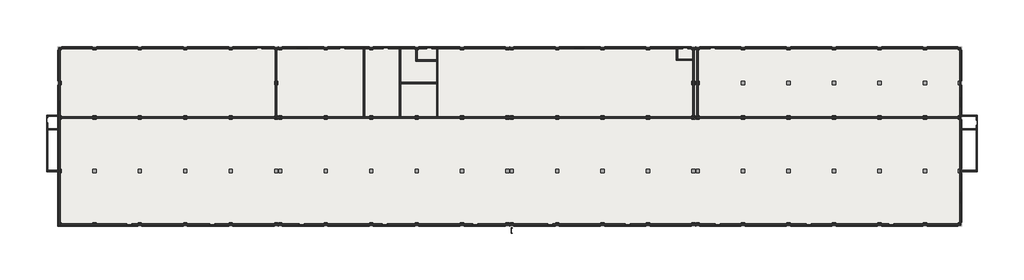
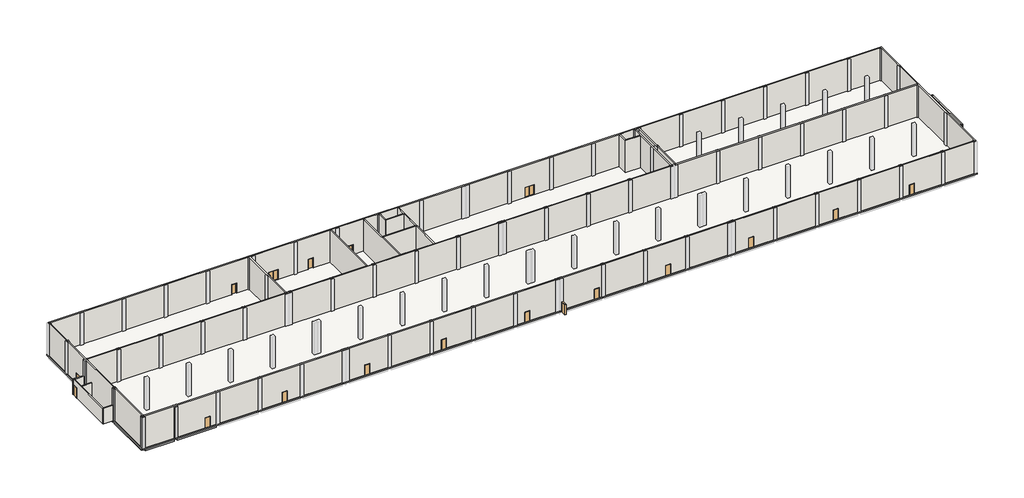
# One storey, part 1 of 4: 27 walls, 24 doors, 4 beams, 4 columns, 1 slab.
"""IFC4 building model written with IfcOpenShell, lengths in millimetres."""

import ifcopenshell
import ifcopenshell.guid

model = None  # the IFC model being written
_history = None  # IfcOwnerHistory: only IFC2X3 demands one
_inside = {}  # id of a spatial element -> (the spatial element, [elements in it])
_under = {}  # id of a project, library or spatial element -> (it, [spatial elements below it])
_declared = {}  # id of a project -> (the project, [libraries it declares])
_typed = {}  # id of a type object -> (the type object, [elements of that type])
_made_of = {}  # id of a material, layer set ... -> (it, [elements and type objects made of it])


def new_model(schema):
    """Start an empty IFC model of exactly this schema.

    Asked for "IFC4X3", IfcOpenShell would pick the latest addendum, in which some entities
    have other attributes; the version numbers below select the first issue.
    IFC2X3 requires an IfcOwnerHistory on every rooted entity: one is made here for all.
    """
    global model, _history
    if schema == "IFC4X3":
        model = ifcopenshell.file(schema_version=(4, 3, 0, 0))
    else:
        model = ifcopenshell.file(schema=schema)
    _inside.clear()
    _under.clear()
    _declared.clear()
    _typed.clear()
    _made_of.clear()
    _history = None
    if model.schema == "IFC2X3":
        org = make("IfcOrganization", Name="unknown")
        user = make(
            "IfcPersonAndOrganization",
            ThePerson=make("IfcPerson", FamilyName="unknown"),
            TheOrganization=org,
        )
        app = make(
            "IfcApplication",
            ApplicationDeveloper=org,
            Version="unknown",
            ApplicationFullName="unknown",
            ApplicationIdentifier="unknown",
        )
        _history = make(
            "IfcOwnerHistory",
            OwningUser=user,
            OwningApplication=app,
            ChangeAction="ADDED",
            CreationDate=0,
        )
    return model


def make(cls, **values):
    """One entity of the class cls with the attributes given. An attribute that is None is left unset."""
    return model.create_entity(
        cls, **{name: value for name, value in values.items() if value is not None}
    )


def rooted(cls, **values):
    """An entity with a GlobalId (a new one), such as an element, a storey or a relation."""
    return make(cls, GlobalId=ifcopenshell.guid.new(), OwnerHistory=_history, **values)


def si_unit(unit_type, name, prefix=None):
    """IfcSIUnit, for example si_unit("LENGTHUNIT", "METRE", prefix="MILLI")."""
    return make("IfcSIUnit", UnitType=unit_type, Prefix=prefix, Name=name)


def assignment(units):
    """IfcUnitAssignment: the units of a project."""
    return None if units is None else make("IfcUnitAssignment", Units=units)


def point(xyz):
    """IfcCartesianPoint."""
    return None if xyz is None else make("IfcCartesianPoint", Coordinates=xyz)


def direction(xyz):
    """IfcDirection."""
    return None if xyz is None else make("IfcDirection", DirectionRatios=xyz)


def frame(location, z_axis=None, x_axis=None):
    """IfcAxis2Placement3D, a coordinate frame: its origin and axes. An axis left out is left unset."""
    return make(
        "IfcAxis2Placement3D",
        Location=point(location),
        Axis=direction(z_axis),
        RefDirection=direction(x_axis),
    )


def origin():
    """The frame at (0, 0, 0) with its axes left unset."""
    return frame((0.0, 0.0, 0.0))


def origin_with_axes():
    """The frame at (0, 0, 0) with the z axis (0, 0, 1) and the x axis (1, 0, 0) written out."""
    return frame((0.0, 0.0, 0.0), z_axis=(0.0, 0.0, 1.0), x_axis=(1.0, 0.0, 0.0))


def place(relative_to, where):
    """IfcLocalPlacement: puts the frame where relative to a parent placement (None: the world)."""
    return make(
        "IfcLocalPlacement", PlacementRelTo=relative_to, RelativePlacement=where
    )


def context(
    kind, dimensions, precision=None, world=None, true_north=None, identifier=None
):
    """IfcGeometricRepresentationContext, for example the 3D "Model" context."""
    return make(
        "IfcGeometricRepresentationContext",
        ContextIdentifier=identifier,
        ContextType=kind,
        CoordinateSpaceDimension=dimensions,
        Precision=precision,
        WorldCoordinateSystem=world,
        TrueNorth=true_north,
    )


def project(units=None, contexts=None):
    """IfcProject with its units and contexts."""
    return rooted(
        "IfcProject",
        Name="project",
        RepresentationContexts=contexts,
        UnitsInContext=assignment(units),
    )


def spatial(cls, under=None, at=None, **own):
    """A site, building, storey or space (cls), placed at a placement, below another one or the project."""
    s = rooted(cls, ObjectPlacement=at, **own)
    if under is not None:
        _under.setdefault(under.id(), (under, []))[1].append(s)
    return s


def polyline(points):
    """IfcPolyline through the points."""
    return make("IfcPolyline", Points=[point(p) for p in points])


def outline(outer, holes=None, kind="AREA"):
    """IfcArbitraryClosedProfileDef: a profile drawn as a closed curve; with holes, ...WithVoids."""
    if holes is None:
        return make("IfcArbitraryClosedProfileDef", ProfileType=kind, OuterCurve=outer)
    return make(
        "IfcArbitraryProfileDefWithVoids",
        ProfileType=kind,
        OuterCurve=outer,
        InnerCurves=holes,
    )


def extrude(swept, where, along, depth):
    """IfcExtrudedAreaSolid: the profile swept, set in the frame where, extruded along a direction by depth."""
    return make(
        "IfcExtrudedAreaSolid",
        SweptArea=swept,
        Position=where,
        ExtrudedDirection=direction(along),
        Depth=depth,
    )


def faces_of(points, faces, orient=None, outer=None):
    """IfcFace entities. A face is a list of loops; a loop is a list of indices into points, from 0.

    orient and outer hold one flag for each loop. By default every Orientation is true, the
    first loop of a face is its IfcFaceOuterBound and the others are IfcFaceBound.
    """
    made = []
    for i, loops in enumerate(faces):
        bounds = []
        for j, loop in enumerate(loops):
            is_outer = j == 0 if outer is None else outer[i][j]
            bounds.append(
                make(
                    "IfcFaceOuterBound" if is_outer else "IfcFaceBound",
                    Bound=make("IfcPolyLoop", Polygon=[points[k] for k in loop]),
                    Orientation=True if orient is None else orient[i][j],
                )
            )
        made.append(make("IfcFace", Bounds=bounds))
    return made


def faceted_brep(points, faces, orient=None, outer=None, voids=None):
    """IfcFacetedBrep: a solid bounded by flat faces; with voids (closed shells), ...WithVoids."""
    shared = [point(p) for p in points]
    hull = make("IfcClosedShell", CfsFaces=faces_of(shared, faces, orient, outer))
    if voids is None:
        return make("IfcFacetedBrep", Outer=hull)
    return make(
        "IfcFacetedBrepWithVoids",
        Outer=hull,
        Voids=[
            make(cls, CfsFaces=faces_of(shared, fs, o, b)) for cls, fs, o, b in voids
        ],
    )


def shape(context_of_items, identifier, shape_type, items):
    """IfcShapeRepresentation: the items that make up one representation, for example the "Body"."""
    return make(
        "IfcShapeRepresentation",
        ContextOfItems=context_of_items,
        RepresentationIdentifier=identifier,
        RepresentationType=shape_type,
        Items=items,
    )


def source(mapping_origin, context_of_items, identifier, shape_type, items):
    """IfcRepresentationMap: a shape defined once, which mapped items show again and again."""
    return make(
        "IfcRepresentationMap",
        MappingOrigin=mapping_origin,
        MappedRepresentation=shape(context_of_items, identifier, shape_type, items),
    )


def transform(
    local_origin,
    x_axis=None,
    y_axis=None,
    z_axis=None,
    scale=None,
    scale2=None,
    scale3=None,
    uniform=True,
):
    """IfcCartesianTransformationOperator3D, or its non-uniform kind. x_axis, y_axis, z_axis: its Axis1, 2, 3."""
    if uniform:
        return make(
            "IfcCartesianTransformationOperator3D",
            Axis1=direction(x_axis),
            Axis2=direction(y_axis),
            LocalOrigin=point(local_origin),
            Scale=scale,
            Axis3=direction(z_axis),
        )
    return make(
        "IfcCartesianTransformationOperator3DnonUniform",
        Axis1=direction(x_axis),
        Axis2=direction(y_axis),
        LocalOrigin=point(local_origin),
        Scale=scale,
        Axis3=direction(z_axis),
        Scale2=scale2,
        Scale3=scale3,
    )


def mapped(mapping_source, mapping_target):
    """IfcMappedItem: shows the shape of a source again, moved by a transform."""
    return make(
        "IfcMappedItem", MappingSource=mapping_source, MappingTarget=mapping_target
    )


def made_of(thing, what):
    """Note that an element or type object is made of a material, layer set ...; save() writes the relation."""
    if what is not None:
        _made_of.setdefault(what.id(), (what, []))[1].append(thing)
    return thing


def element(
    cls,
    number,
    at=None,
    inside=None,
    cuts=None,
    type_object=None,
    material=None,
    context=None,
    identifier="Body",
    shape_type=None,
    held_by="IfcProductDefinitionShape",
    body=None,
    shapes=None,
    **own,
):
    """One element of the class cls, such as IfcWall. Its Tag is "e" and its number.

    at: its placement. inside: the storey or other place that contains it. cuts: it is an
    opening in that element (IfcRelVoidsElement). A single representation is given by context,
    identifier, shape_type and body (its items); several are given by shapes. held_by: the class
    of the entity that holds the representations. save() writes the other relations.
    """
    e = rooted(cls, Tag="e%d" % number, ObjectPlacement=at, **own)
    if body is not None:
        shapes = [shape(context, identifier, shape_type, body)]
    if shapes is not None:
        e.Representation = make(held_by, Representations=shapes)
    if inside is not None:
        _inside.setdefault(inside.id(), (inside, []))[1].append(e)
    if cuts is not None:
        rooted(
            "IfcRelVoidsElement", RelatingBuildingElement=cuts, RelatedOpeningElement=e
        )
    if type_object is not None:
        _typed.setdefault(type_object.id(), (type_object, []))[1].append(e)
    return made_of(e, material)


def aggregate(whole, parts):
    """IfcRelAggregates: a whole, such as a stair, and the parts it consists of."""
    return rooted("IfcRelAggregates", RelatingObject=whole, RelatedObjects=parts)


def save(model, path):
    """Write the relations noted so far, then the file.

    IfcRelAggregates (storeys below a building ...), IfcRelContainedInSpatialStructure (elements
    in a storey), IfcRelDefinesByType, IfcRelAssociatesMaterial and IfcRelDeclares: one each for
    every whole, place, type object, material and project.
    """
    for whole, parts in _under.values():
        aggregate(whole, parts)
    for where, things in _inside.values():
        rooted(
            "IfcRelContainedInSpatialStructure",
            RelatedElements=things,
            RelatingStructure=where,
        )
    for kind, things in _typed.values():
        rooted("IfcRelDefinesByType", RelatedObjects=things, RelatingType=kind)
    for what, things in _made_of.values():
        rooted("IfcRelAssociatesMaterial", RelatedObjects=things, RelatingMaterial=what)
    for by, libraries in _declared.values():
        rooted("IfcRelDeclares", RelatingContext=by, RelatedDefinitions=libraries)
    model.write(path)


def double_door_steel_22a565f0(model_context):
    return source(origin(), model_context, "Body", "SolidModel", [
        extrude(outline(polyline([(880.0, 60.0), (0.0, 60.0), (0.0, 100.0), (880.0, 100.0), (880.0, 60.0)])), frame((0.0, 0.0, 20.0), z_axis=(0.0, 0.0, 1.0), x_axis=(1.0, 0.0, 0.0)), (0.0, 0.0, 1.0), 2060.0),
        extrude(outline(polyline([(0.0, 60.0), (-880.0, 60.0), (-880.0, 100.0), (0.0, 100.0), (0.0, 60.0)])), frame((0.0, 0.0, 20.0), z_axis=(0.0, 0.0, 1.0), x_axis=(1.0, 0.0, 0.0)), (0.0, 0.0, 1.0), 2060.0),
        faceted_brep([(900.0, -100.0, 2100.0), (900.0, 100.0, 2100.0), (-900.0, 100.0, 2100.0), (-900.0, -100.0, 2100.0), (865.0, 60.0, 2065.0), (865.0, -100.0, 2065.0), (-865.0, -100.0, 2065.0), (-865.0, 60.0, 2065.0), (880.0, 100.0, 2080.0), (880.0, 60.0, 2080.0), (-880.0, 60.0, 2080.0), (-880.0, 100.0, 2080.0), (-900.0, 100.0, 0.0), (-900.0, -100.0, 0.0), (-865.0, -100.0, 35.0), (-865.0, 60.0, 35.0), (-880.0, 60.0, 20.0), (-880.0, 100.0, 20.0), (900.0, 100.0, 0.0), (880.0, 100.0, 20.0), (900.0, -100.0, 0.0), (865.0, -100.0, 35.0), (865.0, 60.0, 35.0), (880.0, 60.0, 20.0)], [[[0, 1, 2, 3]], [[4, 5, 6, 7]], [[8, 9, 10, 11]], [[3, 2, 12, 13]], [[7, 6, 14, 15]], [[11, 10, 16, 17]], [[18, 12, 2, 1], [8, 11, 17, 19]], [[13, 12, 18, 20]], [[0, 3, 13, 20], [21, 14, 6, 5]], [[15, 14, 21, 22]], [[23, 16, 10, 9], [4, 7, 15, 22]], [[17, 16, 23, 19]], [[20, 18, 1, 0]], [[22, 21, 5, 4]], [[19, 23, 9, 8]]]),
    ])


def single_door_steel_02f153ad(model_context):
    return source(origin(), model_context, "Body", "SolidModel", [
        extrude(outline(polyline([(470.0, -130.0), (-470.0, -130.0), (-470.0, -95.0), (470.0, -95.0), (470.0, -130.0)])), origin_with_axes(), (0.0, 0.0, 1.0), 2070.0),
        faceted_brep([(470.0, -130.0, 0.0), (470.0, -95.0, 0.0), (450.0, -95.0, 0.0), (450.0, 95.0, 0.0), (470.0, 95.0, 0.0), (470.0, 130.0, 0.0), (500.0, 130.0, 0.0), (500.0, -130.0, 0.0), (500.0, -130.0, 2100.0), (-500.0, -130.0, 2100.0), (-500.0, -130.0, 0.0), (-470.0, -130.0, 0.0), (-470.0, -130.0, 2070.0), (470.0, -130.0, 2070.0), (500.0, 130.0, 2100.0), (470.0, 130.0, 2070.0), (-470.0, 130.0, 2070.0), (-470.0, 130.0, 0.0), (-500.0, 130.0, 0.0), (-500.0, 130.0, 2100.0), (470.0, 95.0, 2070.0), (450.0, 95.0, 2050.0), (-450.0, 95.0, 2050.0), (-450.0, 95.0, 0.0), (-470.0, 95.0, 0.0), (-470.0, 95.0, 2070.0), (450.0, -95.0, 2050.0), (470.0, -95.0, 2070.0), (-470.0, -95.0, 2070.0), (-470.0, -95.0, 0.0), (-450.0, -95.0, 0.0), (-450.0, -95.0, 2050.0)], [[[0, 1, 2, 3, 4, 5, 6, 7]], [[7, 8, 9, 10, 11, 12, 13, 0]], [[6, 14, 8, 7]], [[5, 15, 16, 17, 18, 19, 14, 6]], [[4, 20, 15, 5]], [[3, 21, 22, 23, 24, 25, 20, 4]], [[2, 26, 21, 3]], [[1, 27, 28, 29, 30, 31, 26, 2]], [[0, 13, 27, 1]], [[12, 11, 29, 28]], [[11, 10, 18, 17, 24, 23, 30, 29]], [[19, 18, 10, 9]], [[25, 24, 17, 16]], [[31, 30, 23, 22]], [[14, 19, 9, 8]], [[20, 25, 16, 15]], [[26, 31, 22, 21]], [[13, 12, 28, 27]]]),
    ])


def single_door_steel_4a6c7de9(model_context):
    return source(origin(), model_context, "Body", "SolidModel", [
        extrude(outline(polyline([(470.0, 130.0), (470.0, 95.0), (-470.0, 95.0), (-470.0, 130.0), (470.0, 130.0)])), origin_with_axes(), (0.0, 0.0, 1.0), 2070.0),
        faceted_brep([(470.0, 130.0, 0.0), (500.0, 130.0, 0.0), (500.0, -130.0, 0.0), (470.0, -130.0, 0.0), (470.0, -95.0, 0.0), (450.0, -95.0, 0.0), (450.0, 95.0, 0.0), (470.0, 95.0, 0.0), (470.0, 130.0, 2070.0), (-470.0, 130.0, 2070.0), (-470.0, 130.0, 0.0), (-500.0, 130.0, 0.0), (-500.0, 130.0, 2100.0), (500.0, 130.0, 2100.0), (500.0, -130.0, 2100.0), (-500.0, -130.0, 2100.0), (-500.0, -130.0, 0.0), (-470.0, -130.0, 0.0), (-470.0, -130.0, 2070.0), (470.0, -130.0, 2070.0), (470.0, -95.0, 2070.0), (-470.0, -95.0, 2070.0), (-470.0, -95.0, 0.0), (-450.0, -95.0, 0.0), (-450.0, -95.0, 2050.0), (450.0, -95.0, 2050.0), (450.0, 95.0, 2050.0), (-450.0, 95.0, 2050.0), (-450.0, 95.0, 0.0), (-470.0, 95.0, 0.0), (-470.0, 95.0, 2070.0), (470.0, 95.0, 2070.0)], [[[0, 1, 2, 3, 4, 5, 6, 7]], [[1, 0, 8, 9, 10, 11, 12, 13]], [[2, 1, 13, 14]], [[3, 2, 14, 15, 16, 17, 18, 19]], [[4, 3, 19, 20]], [[5, 4, 20, 21, 22, 23, 24, 25]], [[6, 5, 25, 26]], [[7, 6, 26, 27, 28, 29, 30, 31]], [[0, 7, 31, 8]], [[9, 30, 29, 10]], [[10, 29, 28, 23, 22, 17, 16, 11]], [[15, 12, 11, 16]], [[21, 18, 17, 22]], [[27, 24, 23, 28]], [[14, 13, 12, 15]], [[20, 19, 18, 21]], [[26, 25, 24, 27]], [[8, 31, 30, 9]]]),
    ])


model = new_model("IFC4")

# Units and contexts
model_context = context("Model", 3, world=origin())
ifc_project = project(units=[si_unit("LENGTHUNIT", "METRE", prefix="MILLI")], contexts=[model_context])

# Site, building, storey
site = spatial("IfcSite", under=ifc_project)
building = spatial("IfcBuilding", under=site)
storey = spatial("IfcBuildingStorey", under=building, Name="01_T.O.F", Elevation=299.9618634)

# Beams
placement = place(None, origin())
element("IfcBeam", 1, ObjectType="RC Beam_Rectangular : H_SB_AR_S16_TG_B400xH600", at=placement, inside=storey, context=model_context, shape_type="SweptSolid", body=[
    extrude(outline(polyline([(-4545.0, -6300.4791411), (-4195.0, -6300.4791411), (-4195.0, -15350.4791411), (-4545.0, -15350.4791411), (-4545.0, -6300.4791411)])), frame((0.0, 0.0, -300.0381366), z_axis=(0.0, 0.0, 1.0), x_axis=(1.0, 0.0, 0.0)), (0.0, 0.0, 1.0), 450.0),
])
element("IfcBeam", 2, ObjectType="RC Beam_Rectangular : H_SB_AR_S16_TG_B400xH600", at=placement, inside=storey, context=model_context, shape_type="SweptSolid", body=[
    extrude(outline(polyline([(-4545.0, -15950.4791411), (-4195.0, -15950.4791411), (-4195.0, -25000.4791411), (-4545.0, -25000.4791411), (-4545.0, -15950.4791411)])), frame((0.0, 0.0, -300.0381366), z_axis=(0.0, 0.0, 1.0), x_axis=(1.0, 0.0, 0.0)), (0.0, 0.0, 1.0), 450.0),
])
element("IfcBeam", 3, ObjectType="RC Beam_Rectangular : H_SB_AR_S16_TG_B400xH600", at=placement, inside=storey, context=model_context, shape_type="SweptSolid", body=[
    extrude(outline(polyline([(-4070.0, -25475.4791411), (-4070.0, -25125.4791411), (1630.0, -25125.4791411), (1630.0, -25475.4791411), (-4070.0, -25475.4791411)])), frame((0.0, 0.0, -300.0381366), z_axis=(0.0, 0.0, 1.0), x_axis=(1.0, 0.0, 0.0)), (0.0, 0.0, 1.0), 450.0),
])
element("IfcBeam", 4, ObjectType="RC Beam_Rectangular : H_SB_AR_S16_TG_B400xH600", at=placement, inside=storey, context=model_context, shape_type="SweptSolid", body=[
    extrude(outline(polyline([(2230.0, -25475.4791411), (2230.0, -25125.4791411), (9830.0, -25125.4791411), (9830.0, -25475.4791411), (2230.0, -25475.4791411)])), frame((0.0, 0.0, -300.0381366), z_axis=(0.0, 0.0, 1.0), x_axis=(1.0, 0.0, 0.0)), (0.0, 0.0, 1.0), 450.0),
])

# Columns
element("IfcColumn", 5, ObjectType="RC_Column_Rectangular : H_SC_AR_S15_W600xL600", at=placement, inside=storey, context=model_context, shape_type="Brep", body=[
    faceted_brep([(-4070.0, -5700.4791411, 299.9618634), (-4070.0, -6300.4791411, 299.9618634), (-4670.0, -6300.4791411, 299.9618634), (-4670.0, -5700.4791411, 299.9618634), (-4070.0, -5700.4791411, 6848.9618634), (-4070.0, -5850.4791411, 6848.9618634), (-4070.0, -6150.4791411, 6848.9618634), (-4070.0, -6300.4791411, 6848.9618634), (-4220.0, -6300.4791411, 6848.9618634), (-4520.0, -6300.4791411, 6848.9618634), (-4670.0, -6300.4791411, 6848.9618634), (-4670.0, -5700.4791411, 6848.9618634), (-4520.0, -5700.4791411, 6848.9618634), (-4220.0, -5700.4791411, 6848.9618634)], [[[0, 1, 2, 3]], [[1, 0, 4, 5, 6, 7]], [[2, 1, 7, 8, 9, 10]], [[3, 2, 10, 11]], [[0, 3, 11, 12, 13, 4]], [[7, 6, 5, 4, 13, 12, 11, 10, 9, 8]]]),
])
element("IfcColumn", 6, ObjectType="RC_Column_Rectangular : H_SC_AR_S15_W600xL600", at=placement, inside=storey, context=model_context, shape_type="Brep", body=[
    faceted_brep([(-4070.0, -15350.4791411, 299.9618634), (-4070.0, -15950.4791411, 299.9618634), (-4670.0, -15950.4791411, 299.9618634), (-4670.0, -15350.4791411, 299.9618634), (-4070.0, -15350.4791411, 6848.9618634), (-4070.0, -15500.4791411, 6848.9618634), (-4070.0, -15800.4791411, 6848.9618634), (-4070.0, -15950.4791411, 6848.9618634), (-4220.0, -15950.4791411, 6848.9618634), (-4520.0, -15950.4791411, 6848.9618634), (-4670.0, -15950.4791411, 6848.9618634), (-4670.0, -15350.4791411, 6848.9618634), (-4520.0, -15350.4791411, 6848.9618634), (-4220.0, -15350.4791411, 6848.9618634)], [[[0, 1, 2, 3]], [[1, 0, 4, 5, 6, 7]], [[2, 1, 7, 8, 9, 10]], [[3, 2, 10, 11]], [[0, 3, 11, 12, 13, 4]], [[7, 6, 5, 4, 13, 12, 11, 10, 9, 8]]]),
])
element("IfcColumn", 7, ObjectType="RC_Column_Rectangular : H_SC_AR_S15_W600xL600", at=placement, inside=storey, context=model_context, shape_type="Brep", body=[
    faceted_brep([(-4070.0, -25000.4791411, 299.9618634), (-4070.0, -25600.4791411, 299.9618634), (-4670.0, -25600.4791411, 299.9618634), (-4670.0, -25000.4791411, 299.9618634), (-4070.0, -25000.4791411, 6848.9618634), (-4070.0, -25150.4791411, 6848.9618634), (-4070.0, -25450.4791411, 6848.9618634), (-4070.0, -25600.4791411, 6848.9618634), (-4670.0, -25600.4791411, 6848.9618634), (-4670.0, -25000.4791411, 6848.9618634), (-4520.0, -25000.4791411, 6848.9618634), (-4220.0, -25000.4791411, 6848.9618634)], [[[0, 1, 2, 3]], [[1, 0, 4, 5, 6, 7]], [[2, 1, 7, 8]], [[3, 2, 8, 9]], [[0, 3, 9, 10, 11, 4]], [[7, 6, 5, 4, 11, 10, 9, 8]]]),
])
element("IfcColumn", 8, ObjectType="RC_Column_Rectangular : H_SC_AR_S15_W600xL600", at=placement, inside=storey, context=model_context, shape_type="Brep", body=[
    faceted_brep([(2230.0, -25000.4791411, 299.9618634), (2230.0, -25600.4791411, 299.9618634), (1630.0, -25600.4791411, 299.9618634), (1630.0, -25000.4791411, 299.9618634), (2230.0, -25000.4791411, 6848.9618634), (2230.0, -25150.4791411, 6848.9618634), (2230.0, -25450.4791411, 6848.9618634), (2230.0, -25600.4791411, 6848.9618634), (1630.0, -25600.4791411, 6848.9618634), (1630.0, -25450.4791411, 6848.9618634), (1630.0, -25150.4791411, 6848.9618634), (1630.0, -25000.4791411, 6848.9618634), (1780.0, -25000.4791411, 6848.9618634), (2080.0, -25000.4791411, 6848.9618634)], [[[0, 1, 2, 3]], [[1, 0, 4, 5, 6, 7]], [[2, 1, 7, 8]], [[3, 2, 8, 9, 10, 11]], [[0, 3, 11, 12, 13, 4]], [[7, 6, 5, 4, 13, 12, 11, 10, 9, 8]]]),
])

# Doors
double_door_steel_shape = double_door_steel_22a565f0(model_context)
element("IfcDoor", 9, ObjectType="Double Door_Steel : H_DR_AR_B12_Double Door_Steel_W2000xH2100", at=placement, inside=storey, context=model_context, shape_type="MappedRepresentation", body=[
    mapped(double_door_steel_shape, transform((158130.0, -20481.4791411, 299.9618634), x_axis=(0.0, -1.0, 0.0), y_axis=(1.0, 0.0, 0.0), z_axis=(0.0, 0.0, 1.0))),
])
element("IfcDoor", 10, ObjectType="Double Door_Steel : H_DR_AR_B12_Double Door_Steel_W2000xH2100", at=placement, inside=storey, context=model_context, shape_type="MappedRepresentation", body=[
    mapped(double_door_steel_shape, transform((158130.0, -3288.4791411, 299.9618634), x_axis=(0.0, -1.0, 0.0), y_axis=(1.0, 0.0, 0.0), z_axis=(0.0, 0.0, 1.0))),
])
element("IfcDoor", 11, ObjectType="Double Door_Steel : H_DR_AR_B12_Double Door_Steel_W2000xH2100", at=placement, inside=storey, context=model_context, shape_type="MappedRepresentation", body=[
    mapped(double_door_steel_shape, transform((89423.0, 6499.5208589, 299.9618634), x_axis=(1.0, 0.0, 0.0), y_axis=(0.0, 1.0, 0.0), z_axis=(0.0, 0.0, 1.0))),
])
element("IfcDoor", 12, ObjectType="Double Door_Steel : H_DR_AR_B12_Double Door_Steel_W2000xH2100", at=placement, inside=storey, context=model_context, shape_type="MappedRepresentation", body=[
    mapped(double_door_steel_shape, transform((39442.0, 6499.5208589, 299.9618634), x_axis=(1.0, 0.0, 0.0), y_axis=(0.0, 1.0, 0.0), z_axis=(0.0, 0.0, 1.0))),
])
element("IfcDoor", 13, ObjectType="Double Door_Steel : H_DR_AR_B12_Double Door_Steel_W2000xH2100", at=placement, inside=storey, context=model_context, shape_type="MappedRepresentation", body=[
    mapped(double_door_steel_shape, transform((-4370.0, -3878.4791411, 299.9618634), x_axis=(0.0, 1.0, 0.0), y_axis=(-1.0, 0.0, 0.0), z_axis=(0.0, 0.0, 1.0))),
])
single_door_steel_shape = single_door_steel_02f153ad(model_context)
element("IfcDoor", 14, ObjectType="Single Door_Steel : H_DR_AR_B12_Single Door_Steel_W1000xH2100", at=placement, inside=storey, context=model_context, shape_type="MappedRepresentation", body=[
    mapped(single_door_steel_shape, transform((-6570.0, -6512.4791411, 299.9618634), x_axis=(0.0, -1.0, 0.0), y_axis=(1.0, 0.0, 0.0), z_axis=(0.0, 0.0, 1.0))),
])
element("IfcDoor", 15, ObjectType="Single Door_Steel : H_DR_AR_B12_Single Door_Steel_W1000xH2100", at=placement, inside=storey, context=model_context, shape_type="MappedRepresentation", body=[
    mapped(single_door_steel_shape, transform((8230.0, -25300.4791411, 299.9618634), x_axis=(1.0, 0.0, 0.0), y_axis=(0.0, 1.0, 0.0), z_axis=(0.0, 0.0, 1.0))),
])
element("IfcDoor", 16, ObjectType="Single Door_Steel : H_DR_AR_B12_Single Door_Steel_W1000xH2100", at=placement, inside=storey, context=model_context, shape_type="MappedRepresentation", body=[
    mapped(single_door_steel_shape, transform((23230.0, -25300.4791411, 299.9618634), x_axis=(1.0, 0.0, 0.0), y_axis=(0.0, 1.0, 0.0), z_axis=(0.0, 0.0, 1.0))),
])
element("IfcDoor", 17, ObjectType="Single Door_Steel : H_DR_AR_B12_Single Door_Steel_W1000xH2100", at=placement, inside=storey, context=model_context, shape_type="MappedRepresentation", body=[
    mapped(single_door_steel_shape, transform((39330.0, -25300.4791411, 299.9618634), x_axis=(1.0, 0.0, 0.0), y_axis=(0.0, 1.0, 0.0), z_axis=(0.0, 0.0, 1.0))),
])
element("IfcDoor", 18, ObjectType="Single Door_Steel : H_DR_AR_B12_Single Door_Steel_W1000xH2100", at=placement, inside=storey, context=model_context, shape_type="MappedRepresentation", body=[
    mapped(single_door_steel_shape, transform((54330.0, -25300.4791411, 299.9618634), x_axis=(1.0, 0.0, 0.0), y_axis=(0.0, 1.0, 0.0), z_axis=(0.0, 0.0, 1.0))),
])
element("IfcDoor", 19, ObjectType="Single Door_Steel : H_DR_AR_B12_Single Door_Steel_W1000xH2100", at=placement, inside=storey, context=model_context, shape_type="MappedRepresentation", body=[
    mapped(single_door_steel_shape, transform((70608.0, -25300.4791411, 299.9618634), x_axis=(1.0, 0.0, 0.0), y_axis=(0.0, 1.0, 0.0), z_axis=(0.0, 0.0, 1.0))),
])
element("IfcDoor", 20, ObjectType="Single Door_Steel : H_DR_AR_B12_Single Door_Steel_W1000xH2100", at=placement, inside=storey, context=model_context, shape_type="MappedRepresentation", body=[
    mapped(single_door_steel_shape, transform((77230.0, -26400.4791411, 299.9618634), x_axis=(0.0, -1.0, 0.0), y_axis=(1.0, 0.0, 0.0), z_axis=(0.0, 0.0, 1.0))),
])
element("IfcDoor", 21, ObjectType="Single Door_Steel : H_DR_AR_B12_Single Door_Steel_W1000xH2100", at=placement, inside=storey, context=model_context, shape_type="MappedRepresentation", body=[
    mapped(single_door_steel_shape, transform((84164.0, -25300.4791411, 299.9618634), x_axis=(1.0, 0.0, 0.0), y_axis=(0.0, 1.0, 0.0), z_axis=(0.0, 0.0, 1.0))),
])
element("IfcDoor", 22, ObjectType="Single Door_Steel : H_DR_AR_B12_Single Door_Steel_W1000xH2100", at=placement, inside=storey, context=model_context, shape_type="MappedRepresentation", body=[
    mapped(single_door_steel_shape, transform((98164.0, -25300.4791411, 299.9618634), x_axis=(1.0, 0.0, 0.0), y_axis=(0.0, 1.0, 0.0), z_axis=(0.0, 0.0, 1.0))),
])
element("IfcDoor", 23, ObjectType="Single Door_Steel : H_DR_AR_B12_Single Door_Steel_W1000xH2100", at=placement, inside=storey, context=model_context, shape_type="MappedRepresentation", body=[
    mapped(single_door_steel_shape, transform((114364.0, -25300.4791411, 299.9618634), x_axis=(1.0, 0.0, 0.0), y_axis=(0.0, 1.0, 0.0), z_axis=(0.0, 0.0, 1.0))),
])
element("IfcDoor", 24, ObjectType="Single Door_Steel : H_DR_AR_B12_Single Door_Steel_W1000xH2100", at=placement, inside=storey, context=model_context, shape_type="MappedRepresentation", body=[
    mapped(single_door_steel_shape, transform((130864.0, -25300.4791411, 299.9618634), x_axis=(1.0, 0.0, 0.0), y_axis=(0.0, 1.0, 0.0), z_axis=(0.0, 0.0, 1.0))),
])
element("IfcDoor", 25, ObjectType="Single Door_Steel : H_DR_AR_B12_Single Door_Steel_W1000xH2100", at=placement, inside=storey, context=model_context, shape_type="MappedRepresentation", body=[
    mapped(single_door_steel_shape, transform((145730.0, -25300.4791411, 299.9618634), x_axis=(1.0, 0.0, 0.0), y_axis=(0.0, 1.0, 0.0), z_axis=(0.0, 0.0, 1.0))),
])
element("IfcDoor", 26, ObjectType="Single Door_Steel : H_DR_AR_B12_Single Door_Steel_W1000xH2100", at=placement, inside=storey, context=model_context, shape_type="MappedRepresentation", body=[
    mapped(single_door_steel_shape, transform((113492.0, 6499.5208589, 299.9618634), x_axis=(-1.0, 0.0, 0.0), y_axis=(0.0, -1.0, 0.0), z_axis=(0.0, 0.0, 1.0))),
])
element("IfcDoor", 27, ObjectType="Single Door_Steel : H_DR_AR_B12_Single Door_Steel_W1000xH2100", at=placement, inside=storey, context=model_context, shape_type="MappedRepresentation", body=[
    mapped(single_door_steel_shape, transform((108537.5, 6499.5208589, 299.9618634), x_axis=(-1.0, 0.0, 0.0), y_axis=(0.0, -1.0, 0.0), z_axis=(0.0, 0.0, 1.0))),
])
element("IfcDoor", 28, ObjectType="Single Door_Steel : H_DR_AR_B12_Single Door_Steel_W1000xH2100", at=placement, inside=storey, context=model_context, shape_type="MappedRepresentation", body=[
    mapped(single_door_steel_shape, transform((62358.0, 6499.5208589, 299.9618634), x_axis=(-1.0, 0.0, 0.0), y_axis=(0.0, -1.0, 0.0), z_axis=(0.0, 0.0, 1.0))),
])
element("IfcDoor", 29, ObjectType="Single Door_Steel : H_DR_AR_B12_Single Door_Steel_W1000xH2100", at=placement, inside=storey, context=model_context, shape_type="MappedRepresentation", body=[
    mapped(single_door_steel_shape, transform((54458.0, 6499.5208589, 299.9618634), x_axis=(-1.0, 0.0, 0.0), y_axis=(0.0, -1.0, 0.0), z_axis=(0.0, 0.0, 1.0))),
])
element("IfcDoor", 30, ObjectType="Single Door_Steel : H_DR_AR_B12_Single Door_Steel_W1000xH2100", at=placement, inside=storey, context=model_context, shape_type="MappedRepresentation", body=[
    mapped(single_door_steel_shape, transform((46658.0, 6499.5208589, 299.9618634), x_axis=(-1.0, 0.0, 0.0), y_axis=(0.0, -1.0, 0.0), z_axis=(0.0, 0.0, 1.0))),
])
single_door_steel_2_shape = single_door_steel_4a6c7de9(model_context)
element("IfcDoor", 31, ObjectType="Single Door_Steel : H_DR_AR_B12_Single Door_Steel_W1000xH2100", at=placement, inside=storey, context=model_context, shape_type="MappedRepresentation", body=[
    mapped(single_door_steel_2_shape, transform((31708.0, 6499.5208589, 299.9618634), x_axis=(1.0, 0.0, 0.0), y_axis=(0.0, 1.0, 0.0), z_axis=(0.0, 0.0, 1.0))),
])
element("IfcDoor", 32, ObjectType="Single Door_Steel : H_DR_AR_B12_Single Door_Steel_W1000xH2100", at=placement, inside=storey, context=model_context, shape_type="MappedRepresentation", body=[
    mapped(single_door_steel_2_shape, transform((161130.0, -6922.4791411, 299.9618634), x_axis=(0.0, -1.0, 0.0), y_axis=(1.0, 0.0, 0.0), z_axis=(0.0, 0.0, 1.0))),
])

# Slab
element("IfcSlab", 33, ObjectType="H_FL_AR_S17_RC Slab T150", at=placement, inside=storey, context=model_context, shape_type="SweptSolid", body=[
    extrude(outline(polyline([(158430.0, -25600.4791411), (-4670.0, -25600.4791411), (-4670.0, 6799.5208589), (158430.0, 6799.5208589), (158430.0, -25600.4791411)])), frame((0.0, 0.0, 149.9618634), z_axis=(0.0, 0.0, 1.0), x_axis=(1.0, 0.0, 0.0)), (0.0, 0.0, 1.0), 150.0),
])

# Walls
element("IfcWall", 34, ObjectType="H_WA_AR_B02_Ext Wall_RC T200", at=placement, inside=storey, context=model_context, shape_type="Brep", body=[
    faceted_brep([(158230.0, 6599.5208589, 6949.9618634), (158230.0, -25400.4791411, 6949.9618634), (158230.0, -25400.4791411, 299.9618634), (158230.0, -21381.4791411, 299.9618634), (158230.0, -21381.4791411, 2399.9618634), (158230.0, -19581.4791411, 2399.9618634), (158230.0, -19581.4791411, 299.9618634), (158230.0, -15750.4791411, 299.9618634), (158230.0, -15550.4791411, 299.9618634), (158230.0, -8222.4791411, 299.9618634), (158230.0, -8022.4791411, 299.9618634), (158230.0, -5800.4791411, 299.9618634), (158230.0, -5600.4791411, 299.9618634), (158230.0, -4188.4791411, 299.9618634), (158230.0, -4188.4791411, 2399.9618634), (158230.0, -2388.4791411, 2399.9618634), (158230.0, -2388.4791411, 299.9618634), (158230.0, 6599.5208589, 299.9618634), (158030.0, -25400.4791411, 6949.9618634), (158030.0, -25200.4791411, 6949.9618634), (158030.0, -6122.4791411, 6949.9618634), (158030.0, -5888.4791411, 6949.9618634), (158030.0, 6399.5208589, 6949.9618634), (158030.0, 6599.5208589, 6949.9618634), (158030.0, 6599.5208589, 299.9618634), (158030.0, 6399.5208589, 299.9618634), (158030.0, -2388.4791411, 299.9618634), (158030.0, -2388.4791411, 2399.9618634), (158030.0, -4188.4791411, 2399.9618634), (158030.0, -4188.4791411, 299.9618634), (158030.0, -5888.4791411, 299.9618634), (158030.0, -6122.4791411, 299.9618634), (158030.0, -19581.4791411, 299.9618634), (158030.0, -19581.4791411, 2399.9618634), (158030.0, -21381.4791411, 2399.9618634), (158030.0, -21381.4791411, 299.9618634), (158030.0, -25200.4791411, 299.9618634), (158030.0, -25400.4791411, 299.9618634), (158030.0, -25400.4791411, 3449.9618634)], [[[0, 1, 2, 3, 4, 5, 6, 7, 8, 9, 10, 11, 12, 13, 14, 15, 16, 17]], [[18, 19, 20, 21, 22, 23, 24, 25, 26, 27, 28, 29, 30, 31, 32, 33, 34, 35, 36, 37, 38]], [[24, 17, 16, 26, 25]], [[2, 37, 36, 35, 3]], [[6, 32, 31, 30, 29, 13, 12, 11, 10, 9, 8, 7]], [[1, 0, 23, 22, 21, 20, 19, 18]], [[0, 17, 24, 23]], [[1, 18, 38, 37, 2]], [[34, 4, 3, 35]], [[4, 34, 33, 5]], [[5, 33, 32, 6]], [[28, 14, 13, 29]], [[14, 28, 27, 15]], [[15, 27, 26, 16]]]),
])
element("IfcWall", 35, ObjectType="H_WA_AR_B02_Ext Wall_RC T200", at=placement, inside=storey, context=model_context, shape_type="Brep", body=[
    faceted_brep([(-4470.0, 6599.5208589, 6949.9618634), (158030.0, 6599.5208589, 6949.9618634), (158030.0, 6599.5208589, 299.9618634), (113992.0, 6599.5208589, 299.9618634), (113992.0, 6599.5208589, 2399.9618634), (112992.0, 6599.5208589, 2399.9618634), (112992.0, 6599.5208589, 299.9618634), (109037.5, 6599.5208589, 299.9618634), (109037.5, 6599.5208589, 2399.9618634), (108037.5, 6599.5208589, 2399.9618634), (108037.5, 6599.5208589, 299.9618634), (90323.0, 6599.5208589, 299.9618634), (90323.0, 6599.5208589, 2399.9618634), (88523.0, 6599.5208589, 2399.9618634), (88523.0, 6599.5208589, 299.9618634), (62858.0, 6599.5208589, 299.9618634), (62858.0, 6599.5208589, 2399.9618634), (61858.0, 6599.5208589, 2399.9618634), (61858.0, 6599.5208589, 299.9618634), (54958.0, 6599.5208589, 299.9618634), (54958.0, 6599.5208589, 2399.9618634), (53958.0, 6599.5208589, 2399.9618634), (53958.0, 6599.5208589, 299.9618634), (47158.0, 6599.5208589, 299.9618634), (47158.0, 6599.5208589, 2399.9618634), (46158.0, 6599.5208589, 2399.9618634), (46158.0, 6599.5208589, 299.9618634), (40342.0, 6599.5208589, 299.9618634), (40342.0, 6599.5208589, 2399.9618634), (38542.0, 6599.5208589, 2399.9618634), (38542.0, 6599.5208589, 299.9618634), (32208.0, 6599.5208589, 299.9618634), (32208.0, 6599.5208589, 2399.9618634), (31208.0, 6599.5208589, 2399.9618634), (31208.0, 6599.5208589, 299.9618634), (-4470.0, 6599.5208589, 299.9618634), (158030.0, 6399.5208589, 6949.9618634), (110892.0, 6399.5208589, 6949.9618634), (110658.0, 6399.5208589, 6949.9618634), (110152.0, 6399.5208589, 6949.9618634), (109918.0, 6399.5208589, 6949.9618634), (107157.0, 6399.5208589, 6949.9618634), (106923.0, 6399.5208589, 6949.9618634), (63892.0, 6399.5208589, 6949.9618634), (63658.0, 6399.5208589, 6949.9618634), (60192.0, 6399.5208589, 6949.9618634), (59958.0, 6399.5208589, 6949.9618634), (57192.0, 6399.5208589, 6949.9618634), (56958.0, 6399.5208589, 6949.9618634), (50692.0, 6399.5208589, 6949.9618634), (50458.0, 6399.5208589, 6949.9618634), (34842.0, 6399.5208589, 6949.9618634), (34608.0, 6399.5208589, 6949.9618634), (-4270.0, 6399.5208589, 6949.9618634), (-4470.0, 6399.5208589, 6949.9618634), (-4470.0, 6399.5208589, 299.9618634), (-4270.0, 6399.5208589, 299.9618634), (31208.0, 6399.5208589, 299.9618634), (31208.0, 6399.5208589, 2399.9618634), (32208.0, 6399.5208589, 2399.9618634), (32208.0, 6399.5208589, 299.9618634), (34608.0, 6399.5208589, 299.9618634), (34842.0, 6399.5208589, 299.9618634), (38542.0, 6399.5208589, 299.9618634), (38542.0, 6399.5208589, 2399.9618634), (40342.0, 6399.5208589, 2399.9618634), (40342.0, 6399.5208589, 299.9618634), (46158.0, 6399.5208589, 299.9618634), (46158.0, 6399.5208589, 2399.9618634), (47158.0, 6399.5208589, 2399.9618634), (47158.0, 6399.5208589, 299.9618634), (50458.0, 6399.5208589, 299.9618634), (50692.0, 6399.5208589, 299.9618634), (53958.0, 6399.5208589, 299.9618634), (53958.0, 6399.5208589, 2399.9618634), (54958.0, 6399.5208589, 2399.9618634), (54958.0, 6399.5208589, 299.9618634), (56958.0, 6399.5208589, 299.9618634), (57192.0, 6399.5208589, 299.9618634), (59958.0, 6399.5208589, 299.9618634), (60192.0, 6399.5208589, 299.9618634), (61858.0, 6399.5208589, 299.9618634), (61858.0, 6399.5208589, 2399.9618634), (62858.0, 6399.5208589, 2399.9618634), (62858.0, 6399.5208589, 299.9618634), (63658.0, 6399.5208589, 299.9618634), (63892.0, 6399.5208589, 299.9618634), (88523.0, 6399.5208589, 299.9618634), (88523.0, 6399.5208589, 2399.9618634), (90323.0, 6399.5208589, 2399.9618634), (90323.0, 6399.5208589, 299.9618634), (106923.0, 6399.5208589, 299.9618634), (107157.0, 6399.5208589, 299.9618634), (108037.5, 6399.5208589, 299.9618634), (108037.5, 6399.5208589, 2399.9618634), (109037.5, 6399.5208589, 2399.9618634), (109037.5, 6399.5208589, 299.9618634), (109918.0, 6399.5208589, 299.9618634), (110152.0, 6399.5208589, 299.9618634), (110658.0, 6399.5208589, 299.9618634), (110892.0, 6399.5208589, 299.9618634), (112992.0, 6399.5208589, 299.9618634), (112992.0, 6399.5208589, 2399.9618634), (113992.0, 6399.5208589, 2399.9618634), (113992.0, 6399.5208589, 299.9618634), (158030.0, 6399.5208589, 299.9618634)], [[[0, 1, 2, 3, 4, 5, 6, 7, 8, 9, 10, 11, 12, 13, 14, 15, 16, 17, 18, 19, 20, 21, 22, 23, 24, 25, 26, 27, 28, 29, 30, 31, 32, 33, 34, 35]], [[36, 37, 38, 39, 40, 41, 42, 43, 44, 45, 46, 47, 48, 49, 50, 51, 52, 53, 54, 55, 56, 57, 58, 59, 60, 61, 62, 63, 64, 65, 66, 67, 68, 69, 70, 71, 72, 73, 74, 75, 76, 77, 78, 79, 80, 81, 82, 83, 84, 85, 86, 87, 88, 89, 90, 91, 92, 93, 94, 95, 96, 97, 98, 99, 100, 101, 102, 103, 104, 105]], [[2, 105, 104, 3]], [[55, 35, 34, 57, 56]], [[6, 101, 100, 99, 98, 97, 96, 7]], [[10, 93, 92, 91, 90, 11]], [[14, 87, 86, 85, 84, 15]], [[18, 81, 80, 79, 78, 77, 76, 19]], [[22, 73, 72, 71, 70, 23]], [[26, 67, 66, 27]], [[30, 63, 62, 61, 60, 31]], [[1, 0, 54, 53, 52, 51, 50, 49, 48, 47, 46, 45, 44, 43, 42, 41, 40, 39, 38, 37, 36]], [[2, 1, 36, 105]], [[0, 35, 55, 54]], [[6, 5, 102, 101]], [[5, 4, 103, 102]], [[4, 3, 104, 103]], [[10, 9, 94, 93]], [[9, 8, 95, 94]], [[8, 7, 96, 95]], [[89, 12, 11, 90]], [[12, 89, 88, 13]], [[13, 88, 87, 14]], [[18, 17, 82, 81]], [[17, 16, 83, 82]], [[16, 15, 84, 83]], [[22, 21, 74, 73]], [[21, 20, 75, 74]], [[20, 19, 76, 75]], [[26, 25, 68, 67]], [[25, 24, 69, 68]], [[24, 23, 70, 69]], [[65, 28, 27, 66]], [[28, 65, 64, 29]], [[29, 64, 63, 30]], [[59, 32, 31, 60]], [[32, 59, 58, 33]], [[33, 58, 57, 34]]]),
])
element("IfcWall", 36, ObjectType="H_WA_AR_B02_Ext Wall_RC T200", at=placement, inside=storey, context=model_context, shape_type="Brep", body=[
    faceted_brep([(-4470.0, -25400.4791411, 6949.9618634), (-4470.0, 6399.5208589, 6949.9618634), (-4470.0, 6399.5208589, 299.9618634), (-4470.0, -2978.4791411, 299.9618634), (-4470.0, -2978.4791411, 2399.9618634), (-4470.0, -4778.4791411, 2399.9618634), (-4470.0, -4778.4791411, 299.9618634), (-4470.0, -5600.4791411, 299.9618634), (-4470.0, -5800.4791411, 299.9618634), (-4470.0, -8022.4791411, 299.9618634), (-4470.0, -8222.4791411, 299.9618634), (-4470.0, -15550.4791411, 299.9618634), (-4470.0, -15750.4791411, 299.9618634), (-4470.0, -25400.4791411, 299.9618634), (-4270.0, 6399.5208589, 6949.9618634), (-4270.0, -5888.4791411, 6949.9618634), (-4270.0, -6122.4791411, 6949.9618634), (-4270.0, -25200.4791411, 6949.9618634), (-4270.0, -25400.4791411, 6949.9618634), (-4270.0, -25400.4791411, 3449.9618634), (-4270.0, -25400.4791411, 299.9618634), (-4270.0, -25200.4791411, 299.9618634), (-4270.0, -6122.4791411, 299.9618634), (-4270.0, -5888.4791411, 299.9618634), (-4270.0, -4778.4791411, 299.9618634), (-4270.0, -4778.4791411, 2399.9618634), (-4270.0, -2978.4791411, 2399.9618634), (-4270.0, -2978.4791411, 299.9618634), (-4270.0, 6399.5208589, 299.9618634)], [[[0, 1, 2, 3, 4, 5, 6, 7, 8, 9, 10, 11, 12, 13]], [[14, 15, 16, 17, 18, 19, 20, 21, 22, 23, 24, 25, 26, 27, 28]], [[2, 28, 27, 3]], [[20, 13, 12, 11, 10, 9, 8, 7, 6, 24, 23, 22, 21]], [[1, 0, 18, 17, 16, 15, 14]], [[2, 1, 14, 28]], [[18, 0, 13, 20, 19]], [[26, 4, 3, 27]], [[4, 26, 25, 5]], [[5, 25, 24, 6]]]),
])
element("IfcWall", 37, ObjectType="H_WA_AR_B02_Int Wall_Block T200", at=placement, inside=storey, context=model_context, shape_type="Brep", body=[
    faceted_brep([(34608.0, 6399.5208589, 299.9618634), (34608.0, -5888.4791411, 299.9618634), (34608.0, -6122.4791411, 299.9618634), (34608.0, -6122.4791411, 6949.9618634), (34608.0, -5888.4791411, 6949.9618634), (34608.0, 6399.5208589, 6949.9618634), (34842.0, 6399.5208589, 299.9618634), (34842.0, 6399.5208589, 6949.9618634), (34842.0, -5888.4791411, 6949.9618634), (34842.0, -6122.4791411, 6949.9618634), (34842.0, -6122.4791411, 299.9618634), (34842.0, -5888.4791411, 299.9618634)], [[[0, 1, 2, 3, 4, 5]], [[6, 7, 8, 9, 10, 11]], [[2, 1, 0, 6, 11, 10]], [[5, 4, 3, 9, 8, 7]], [[0, 5, 7, 6]], [[3, 2, 10, 9]]]),
])
element("IfcWall", 38, ObjectType="H_WA_AR_B02_Int Wall_Block T200", at=placement, inside=storey, context=model_context, shape_type="SweptSolid", body=[
    extrude(outline(polyline([(-4270.0, -5888.4791411), (34608.0, -5888.4791411), (34608.0, -6122.4791411), (-4270.0, -6122.4791411), (-4270.0, -5888.4791411)])), frame((0.0, 0.0, 299.9618634), z_axis=(0.0, 0.0, 1.0), x_axis=(1.0, 0.0, 0.0)), (0.0, 0.0, 1.0), 6650.0),
])
element("IfcWall", 39, ObjectType="H_WA_AR_B02_Int Wall_Block T200", at=placement, inside=storey, context=model_context, shape_type="Brep", body=[
    faceted_brep([(35480.0, -6122.4791411, 299.9618634), (110152.0, -6122.4791411, 299.9618634), (110152.0, -6122.4791411, 6949.9618634), (35480.0, -6122.4791411, 6949.9618634), (35480.0, -5888.4791411, 299.9618634), (35480.0, -5888.4791411, 6949.9618634), (50458.0, -5888.4791411, 6949.9618634), (50692.0, -5888.4791411, 6949.9618634), (56958.0, -5888.4791411, 6949.9618634), (57192.0, -5888.4791411, 6949.9618634), (63658.0, -5888.4791411, 6949.9618634), (63892.0, -5888.4791411, 6949.9618634), (109918.0, -5888.4791411, 6949.9618634), (110152.0, -5888.4791411, 6949.9618634), (110152.0, -5888.4791411, 299.9618634), (109918.0, -5888.4791411, 299.9618634), (63892.0, -5888.4791411, 299.9618634), (63658.0, -5888.4791411, 299.9618634), (57192.0, -5888.4791411, 299.9618634), (56958.0, -5888.4791411, 299.9618634), (50692.0, -5888.4791411, 299.9618634), (50458.0, -5888.4791411, 299.9618634)], [[[0, 1, 2, 3]], [[4, 5, 6, 7, 8, 9, 10, 11, 12, 13, 14, 15, 16, 17, 18, 19, 20, 21]], [[1, 0, 4, 21, 20, 19, 18, 17, 16, 15, 14]], [[3, 2, 13, 12, 11, 10, 9, 8, 7, 6, 5]], [[0, 3, 5, 4]], [[2, 1, 14, 13]]]),
])
element("IfcWall", 40, ObjectType="H_WA_AR_B02_Int Wall_Block T200", at=placement, inside=storey, context=model_context, shape_type="Brep", body=[
    faceted_brep([(110152.0, -5888.4791411, 299.9618634), (110152.0, 6399.5208589, 299.9618634), (110152.0, 6399.5208589, 6949.9618634), (110152.0, -5888.4791411, 6949.9618634), (109918.0, -5888.4791411, 299.9618634), (109918.0, -5888.4791411, 6949.9618634), (109918.0, 4287.5208589, 6949.9618634), (109918.0, 4521.5208589, 6949.9618634), (109918.0, 6399.5208589, 6949.9618634), (109918.0, 6399.5208589, 299.9618634), (109918.0, 4521.5208589, 299.9618634), (109918.0, 4287.5208589, 299.9618634)], [[[0, 1, 2, 3]], [[4, 5, 6, 7, 8, 9, 10, 11]], [[1, 0, 4, 11, 10, 9]], [[3, 2, 8, 7, 6, 5]], [[0, 3, 5, 4]], [[2, 1, 9, 8]]]),
])
element("IfcWall", 41, ObjectType="H_WA_AR_B02_Int Wall_Block T200", at=placement, inside=storey, context=model_context, shape_type="Brep", body=[
    faceted_brep([(109918.0, 4521.5208589, 299.9618634), (107157.0, 4521.5208589, 299.9618634), (106923.0, 4521.5208589, 299.9618634), (106923.0, 4521.5208589, 6949.9618634), (107157.0, 4521.5208589, 6949.9618634), (109918.0, 4521.5208589, 6949.9618634), (109918.0, 4287.5208589, 299.9618634), (109918.0, 4287.5208589, 6949.9618634), (106923.0, 4287.5208589, 6949.9618634), (106923.0, 4287.5208589, 299.9618634)], [[[0, 1, 2, 3, 4, 5]], [[6, 7, 8, 9]], [[2, 1, 0, 6, 9]], [[5, 4, 3, 8, 7]], [[0, 5, 7, 6]], [[3, 2, 9, 8]]]),
])
element("IfcWall", 42, ObjectType="H_WA_AR_B02_Int Wall_Block T200", at=placement, inside=storey, context=model_context, shape_type="SweptSolid", body=[
    extrude(outline(polyline([(107157.0, 6399.5208589), (107157.0, 4521.5208589), (106923.0, 4521.5208589), (106923.0, 6399.5208589), (107157.0, 6399.5208589)])), frame((0.0, 0.0, 299.9618634), z_axis=(0.0, 0.0, 1.0), x_axis=(1.0, 0.0, 0.0)), (0.0, 0.0, 1.0), 6650.0),
])
element("IfcWall", 43, ObjectType="H_WA_AR_B02_Int Wall_Block T200", at=placement, inside=storey, context=model_context, shape_type="Brep", body=[
    faceted_brep([(110658.0, -6122.4791411, 299.9618634), (158030.0, -6122.4791411, 299.9618634), (158030.0, -6122.4791411, 6949.9618634), (110658.0, -6122.4791411, 6949.9618634), (110658.0, -5888.4791411, 299.9618634), (110658.0, -5888.4791411, 6949.9618634), (110892.0, -5888.4791411, 6949.9618634), (158030.0, -5888.4791411, 6949.9618634), (158030.0, -5888.4791411, 299.9618634), (110892.0, -5888.4791411, 299.9618634)], [[[0, 1, 2, 3]], [[4, 5, 6, 7, 8, 9]], [[1, 0, 4, 9, 8]], [[3, 2, 7, 6, 5]], [[2, 1, 8, 7]], [[0, 3, 5, 4]]]),
])
element("IfcWall", 44, ObjectType="H_WA_AR_B02_Ext Wall_RC T200", at=placement, inside=storey, context=model_context, shape_type="Brep", body=[
    faceted_brep([(158230.0, -5800.4791411, 299.9618634), (161030.0, -5800.4791411, 299.9618634), (161230.0, -5800.4791411, 299.9618634), (161230.0, -5800.4791411, 3449.9618634), (161030.0, -5800.4791411, 3449.9618634), (158230.0, -5800.4791411, 3449.9618634), (158230.0, -5600.4791411, 299.9618634), (158230.0, -5600.4791411, 3449.9618634), (161230.0, -5600.4791411, 3449.9618634), (161230.0, -5600.4791411, 299.9618634)], [[[0, 1, 2, 3, 4, 5]], [[6, 7, 8, 9]], [[2, 1, 0, 6, 9]], [[5, 4, 3, 8, 7]], [[3, 2, 9, 8]], [[0, 5, 7, 6]]]),
])
element("IfcWall", 45, ObjectType="H_WA_AR_B02_Ext Wall_RC T200", at=placement, inside=storey, context=model_context, shape_type="Brep", body=[
    faceted_brep([(161030.0, -15750.4791411, 3449.9618634), (161030.0, -15550.4791411, 3449.9618634), (161030.0, -8222.4791411, 3449.9618634), (161030.0, -8022.4791411, 3449.9618634), (161030.0, -5800.4791411, 3449.9618634), (161030.0, -5800.4791411, 299.9618634), (161030.0, -6422.4791411, 299.9618634), (161030.0, -6422.4791411, 2399.9618634), (161030.0, -7422.4791411, 2399.9618634), (161030.0, -7422.4791411, 299.9618634), (161030.0, -8022.4791411, 299.9618634), (161030.0, -8222.4791411, 299.9618634), (161030.0, -15550.4791411, 299.9618634), (161030.0, -15750.4791411, 299.9618634), (161230.0, -5800.4791411, 3449.9618634), (161230.0, -15750.4791411, 3449.9618634), (161230.0, -15750.4791411, 299.9618634), (161230.0, -7422.4791411, 299.9618634), (161230.0, -7422.4791411, 2399.9618634), (161230.0, -6422.4791411, 2399.9618634), (161230.0, -6422.4791411, 299.9618634), (161230.0, -5800.4791411, 299.9618634)], [[[0, 1, 2, 3, 4, 5, 6, 7, 8, 9, 10, 11, 12, 13]], [[14, 15, 16, 17, 18, 19, 20, 21]], [[5, 21, 20, 6]], [[16, 13, 12, 11, 10, 9, 17]], [[4, 3, 2, 1, 0, 15, 14]], [[5, 4, 14, 21]], [[0, 13, 16, 15]], [[8, 18, 17, 9]], [[18, 8, 7, 19]], [[19, 7, 6, 20]]]),
])
element("IfcWall", 46, ObjectType="H_WA_AR_B02_Ext Wall_RC T200", at=placement, inside=storey, context=model_context, shape_type="SweptSolid", body=[
    extrude(outline(polyline([(158230.0, -15550.4791411), (161030.0, -15550.4791411), (161030.0, -15750.4791411), (158230.0, -15750.4791411), (158230.0, -15550.4791411)])), frame((0.0, 0.0, 299.9618634), z_axis=(0.0, 0.0, 1.0), x_axis=(1.0, 0.0, 0.0)), (0.0, 0.0, 1.0), 3150.0),
])
element("IfcWall", 47, ObjectType="H_WA_AR_B02_Int Wall_Block T200", at=placement, inside=storey, context=model_context, shape_type="SweptSolid", body=[
    extrude(outline(polyline([(110658.0, -5888.4791411), (110658.0, 6399.5208589), (110892.0, 6399.5208589), (110892.0, -5888.4791411), (110658.0, -5888.4791411)])), frame((0.0, 0.0, 299.9618634), z_axis=(0.0, 0.0, 1.0), x_axis=(1.0, 0.0, 0.0)), (0.0, 0.0, 1.0), 6650.0),
])
element("IfcWall", 48, ObjectType="H_WA_AR_B02_Int Wall_Block T200", at=placement, inside=storey, context=model_context, shape_type="SweptSolid", body=[
    extrude(outline(polyline([(34842.0, -5888.4791411), (35480.0, -5888.4791411), (35480.0, -6122.4791411), (34842.0, -6122.4791411), (34842.0, -5888.4791411)])), frame((0.0, 0.0, 299.9618634), z_axis=(0.0, 0.0, 1.0), x_axis=(1.0, 0.0, 0.0)), (0.0, 0.0, 1.0), 6650.0),
])
element("IfcWall", 49, ObjectType="H_WA_AR_B02_Int Wall_Block T200", at=placement, inside=storey, context=model_context, shape_type="SweptSolid", body=[
    extrude(outline(polyline([(50458.0, -5888.4791411), (50458.0, 6399.5208589), (50692.0, 6399.5208589), (50692.0, -5888.4791411), (50458.0, -5888.4791411)])), frame((0.0, 0.0, 299.9618634), z_axis=(0.0, 0.0, 1.0), x_axis=(1.0, 0.0, 0.0)), (0.0, 0.0, 1.0), 6650.0),
])
element("IfcWall", 50, ObjectType="H_WA_AR_B02_Int Wall_Block T200", at=placement, inside=storey, context=model_context, shape_type="Brep", body=[
    faceted_brep([(56958.0, 6399.5208589, 299.9618634), (56958.0, -5888.4791411, 299.9618634), (56958.0, -5888.4791411, 6949.9618634), (56958.0, 6399.5208589, 6949.9618634), (57192.0, 6399.5208589, 299.9618634), (57192.0, 6399.5208589, 6949.9618634), (57192.0, 359.0208589, 6949.9618634), (57192.0, 125.0208589, 6949.9618634), (57192.0, -5888.4791411, 6949.9618634), (57192.0, -5888.4791411, 299.9618634), (57192.0, 125.0208589, 299.9618634), (57192.0, 359.0208589, 299.9618634)], [[[0, 1, 2, 3]], [[4, 5, 6, 7, 8, 9, 10, 11]], [[1, 0, 4, 11, 10, 9]], [[3, 2, 8, 7, 6, 5]], [[0, 3, 5, 4]], [[2, 1, 9, 8]]]),
])
element("IfcWall", 51, ObjectType="H_WA_AR_B02_Int Wall_Block T200", at=placement, inside=storey, context=model_context, shape_type="Brep", body=[
    faceted_brep([(63658.0, 6399.5208589, 299.9618634), (63658.0, 4411.5208589, 299.9618634), (63658.0, 4177.5208589, 299.9618634), (63658.0, 359.0208589, 299.9618634), (63658.0, 125.0208589, 299.9618634), (63658.0, -5888.4791411, 299.9618634), (63658.0, -5888.4791411, 6949.9618634), (63658.0, 125.0208589, 6949.9618634), (63658.0, 359.0208589, 6949.9618634), (63658.0, 4177.5208589, 6949.9618634), (63658.0, 4411.5208589, 6949.9618634), (63658.0, 6399.5208589, 6949.9618634), (63892.0, 6399.5208589, 299.9618634), (63892.0, 6399.5208589, 6949.9618634), (63892.0, -5888.4791411, 6949.9618634), (63892.0, -5888.4791411, 299.9618634)], [[[0, 1, 2, 3, 4, 5, 6, 7, 8, 9, 10, 11]], [[12, 13, 14, 15]], [[5, 4, 3, 2, 1, 0, 12, 15]], [[11, 10, 9, 8, 7, 6, 14, 13]], [[0, 11, 13, 12]], [[6, 5, 15, 14]]]),
])
element("IfcWall", 52, ObjectType="H_WA_AR_B02_Int Wall_Block T200", at=placement, inside=storey, context=model_context, shape_type="Brep", body=[
    faceted_brep([(59958.0, 6399.5208589, 299.9618634), (59958.0, 4177.5208589, 299.9618634), (59958.0, 4177.5208589, 6949.9618634), (59958.0, 6399.5208589, 6949.9618634), (60192.0, 6399.5208589, 299.9618634), (60192.0, 6399.5208589, 6949.9618634), (60192.0, 4411.5208589, 6949.9618634), (60192.0, 4177.5208589, 6949.9618634), (60192.0, 4177.5208589, 299.9618634), (60192.0, 4411.5208589, 299.9618634)], [[[0, 1, 2, 3]], [[4, 5, 6, 7, 8, 9]], [[1, 0, 4, 9, 8]], [[3, 2, 7, 6, 5]], [[0, 3, 5, 4]], [[2, 1, 8, 7]]]),
])
element("IfcWall", 53, ObjectType="H_WA_AR_B02_Int Wall_Block T200", at=placement, inside=storey, context=model_context, shape_type="SweptSolid", body=[
    extrude(outline(polyline([(63658.0, 4177.5208589), (60192.0, 4177.5208589), (60192.0, 4411.5208589), (63658.0, 4411.5208589), (63658.0, 4177.5208589)])), frame((0.0, 0.0, 299.9618634), z_axis=(0.0, 0.0, 1.0), x_axis=(1.0, 0.0, 0.0)), (0.0, 0.0, 1.0), 6650.0),
])
element("IfcWall", 54, ObjectType="H_WA_AR_B02_Int Wall_Block T200", at=placement, inside=storey, context=model_context, shape_type="SweptSolid", body=[
    extrude(outline(polyline([(63658.0, 125.0208589), (57192.0, 125.0208589), (57192.0, 359.0208589), (63658.0, 359.0208589), (63658.0, 125.0208589)])), frame((0.0, 0.0, 299.9618634), z_axis=(0.0, 0.0, 1.0), x_axis=(1.0, 0.0, 0.0)), (0.0, 0.0, 1.0), 6650.0),
])
element("IfcWall", 55, ObjectType="H_WA_AR_B02_Ext Wall_RC T200", at=placement, inside=storey, context=model_context, shape_type="Brep", body=[
    faceted_brep([(-4470.0, -5600.4791411, 299.9618634), (-6670.0, -5600.4791411, 299.9618634), (-6670.0, -5600.4791411, 3449.9618634), (-4470.0, -5600.4791411, 3449.9618634), (-4470.0, -5800.4791411, 299.9618634), (-4470.0, -5800.4791411, 3449.9618634), (-6470.0, -5800.4791411, 3449.9618634), (-6670.0, -5800.4791411, 3449.9618634), (-6670.0, -5800.4791411, 299.9618634), (-6470.0, -5800.4791411, 299.9618634)], [[[0, 1, 2, 3]], [[4, 5, 6, 7, 8, 9]], [[1, 0, 4, 9, 8]], [[3, 2, 7, 6, 5]], [[0, 3, 5, 4]], [[2, 1, 8, 7]]]),
])
element("IfcWall", 56, ObjectType="H_WA_AR_B02_Ext Wall_RC T200", at=placement, inside=storey, context=model_context, shape_type="Brep", body=[
    faceted_brep([(-6670.0, -15750.4791411, 3449.9618634), (-6670.0, -5800.4791411, 3449.9618634), (-6670.0, -5800.4791411, 299.9618634), (-6670.0, -6012.4791411, 299.9618634), (-6670.0, -6012.4791411, 2399.9618634), (-6670.0, -7012.4791411, 2399.9618634), (-6670.0, -7012.4791411, 299.9618634), (-6670.0, -15750.4791411, 299.9618634), (-6470.0, -5800.4791411, 3449.9618634), (-6470.0, -8022.4791411, 3449.9618634), (-6470.0, -8222.4791411, 3449.9618634), (-6470.0, -15550.4791411, 3449.9618634), (-6470.0, -15750.4791411, 3449.9618634), (-6470.0, -15750.4791411, 299.9618634), (-6470.0, -15550.4791411, 299.9618634), (-6470.0, -8222.4791411, 299.9618634), (-6470.0, -8022.4791411, 299.9618634), (-6470.0, -7012.4791411, 299.9618634), (-6470.0, -7012.4791411, 2399.9618634), (-6470.0, -6012.4791411, 2399.9618634), (-6470.0, -6012.4791411, 299.9618634), (-6470.0, -5800.4791411, 299.9618634)], [[[0, 1, 2, 3, 4, 5, 6, 7]], [[8, 9, 10, 11, 12, 13, 14, 15, 16, 17, 18, 19, 20, 21]], [[2, 21, 20, 3]], [[13, 7, 6, 17, 16, 15, 14]], [[1, 0, 12, 11, 10, 9, 8]], [[2, 1, 8, 21]], [[0, 7, 13, 12]], [[5, 18, 17, 6]], [[18, 5, 4, 19]], [[19, 4, 3, 20]]]),
])
element("IfcWall", 57, ObjectType="H_WA_AR_B02_Ext Wall_RC T200", at=placement, inside=storey, context=model_context, shape_type="SweptSolid", body=[
    extrude(outline(polyline([(-4470.0, -15750.4791411), (-6470.0, -15750.4791411), (-6470.0, -15550.4791411), (-4470.0, -15550.4791411), (-4470.0, -15750.4791411)])), frame((0.0, 0.0, 299.9618634), z_axis=(0.0, 0.0, 1.0), x_axis=(1.0, 0.0, 0.0)), (0.0, 0.0, 1.0), 3150.0),
])
element("IfcWall", 58, ObjectType="H_WA_AR_B02_Ext Wall_RC T200", at=placement, inside=storey, context=model_context, shape_type="SweptSolid", body=[
    extrude(outline(polyline([(6949.9618634, 158030.0), (6949.9618634, -4270.0), (299.9618634, -4270.0), (299.9618634, 7730.0), (2399.9618634, 7730.0), (2399.9618634, 8730.0), (299.9618634, 8730.0), (299.9618634, 22730.0), (2399.9618634, 22730.0), (2399.9618634, 23730.0), (299.9618634, 23730.0), (299.9618634, 38830.0), (2399.9618634, 38830.0), (2399.9618634, 39830.0), (299.9618634, 39830.0), (299.9618634, 53830.0), (2399.9618634, 53830.0), (2399.9618634, 54830.0), (299.9618634, 54830.0), (299.9618634, 70108.0), (2399.9618634, 70108.0), (2399.9618634, 71108.0), (299.9618634, 71108.0), (299.9618634, 83664.0), (2399.9618634, 83664.0), (2399.9618634, 84664.0), (299.9618634, 84664.0), (299.9618634, 97664.0), (2399.9618634, 97664.0), (2399.9618634, 98664.0), (299.9618634, 98664.0), (299.9618634, 113864.0), (2399.9618634, 113864.0), (2399.9618634, 114864.0), (299.9618634, 114864.0), (299.9618634, 130364.0), (2399.9618634, 130364.0), (2399.9618634, 131364.0), (299.9618634, 131364.0), (299.9618634, 145230.0), (2399.9618634, 145230.0), (2399.9618634, 146230.0), (299.9618634, 146230.0), (299.9618634, 158030.0), (6949.9618634, 158030.0)])), frame((0.0, -25400.4791411, 0.0), z_axis=(0.0, 1.0, 0.0), x_axis=(0.0, 0.0, 1.0)), (0.0, 0.0, 1.0), 200.0),
])
element("IfcWall", 59, ObjectType="H_WA_AR_B02_Ext Wall_RC T200", at=placement, inside=storey, context=model_context, shape_type="SweptSolid", body=[
    extrude(outline(polyline([(-4470.0, -8222.4791411), (-6470.0, -8222.4791411), (-6470.0, -8022.4791411), (-4470.0, -8022.4791411), (-4470.0, -8222.4791411)])), frame((0.0, 0.0, 299.9618634), z_axis=(0.0, 0.0, 1.0), x_axis=(1.0, 0.0, 0.0)), (0.0, 0.0, 1.0), 3150.0),
])
element("IfcWall", 60, ObjectType="H_WA_AR_B02_Ext Wall_RC T200", at=placement, inside=storey, context=model_context, shape_type="SweptSolid", body=[
    extrude(outline(polyline([(161030.0, -8222.4791411), (158230.0, -8222.4791411), (158230.0, -8022.4791411), (161030.0, -8022.4791411), (161030.0, -8222.4791411)])), frame((0.0, 0.0, 299.9618634), z_axis=(0.0, 0.0, 1.0), x_axis=(1.0, 0.0, 0.0)), (0.0, 0.0, 1.0), 3150.0),
])

save(model, "model.ifc")
